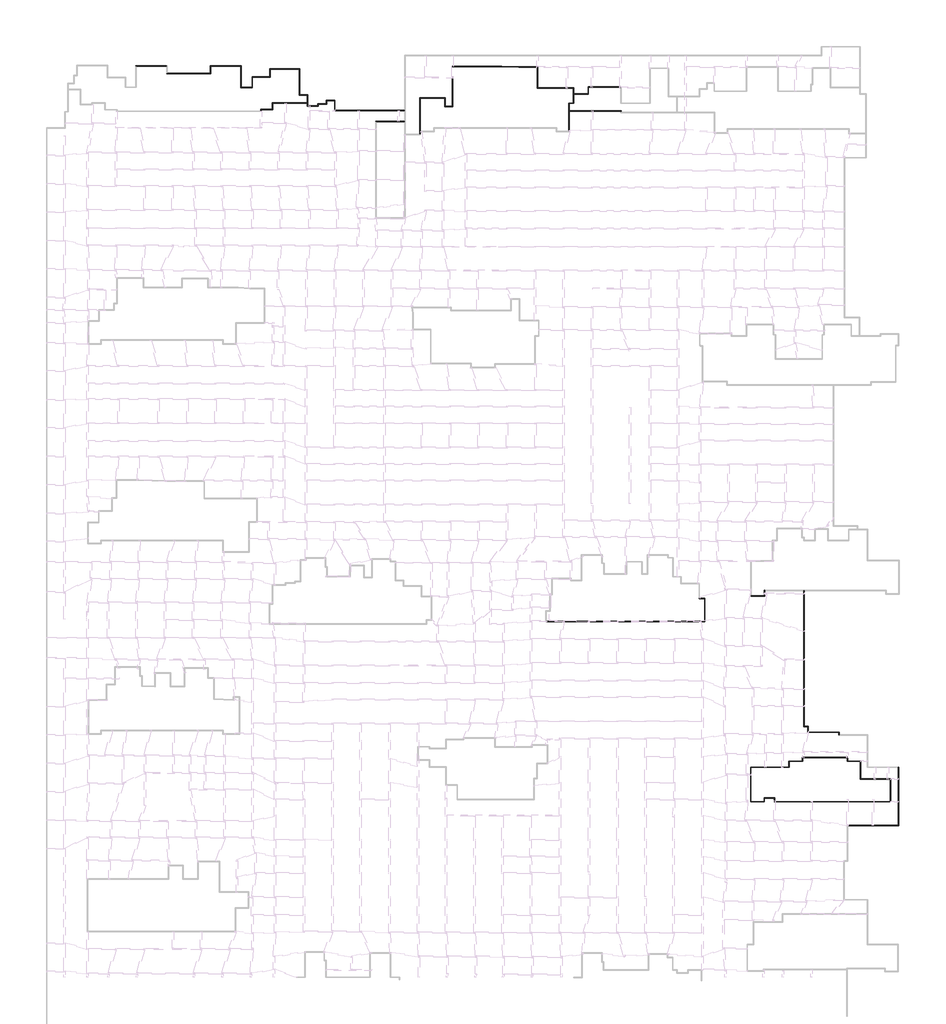
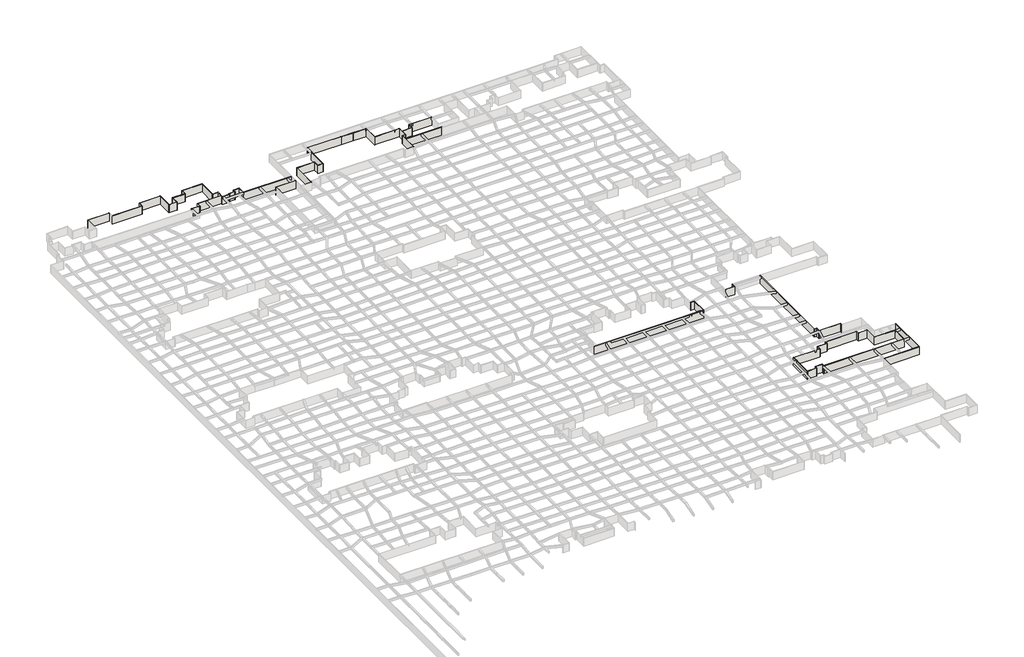
# One storey, part 8 of 45: 70 walls.
"""IFC4 building model written with IfcOpenShell, lengths in millimetres."""

from ifc_helpers import new_model, si_unit, origin, origin_with_axes, place, context, project, spatial, polyline, outline, extrude, faceted_brep, element, save

model = new_model("IFC4")

# Units and contexts
model_context = context("Model", 3, world=origin())
ifc_project = project(units=[si_unit("LENGTHUNIT", "METRE", prefix="MILLI")], contexts=[model_context])

# Site, building, storey
site = spatial("IfcSite", under=ifc_project)
building = spatial("IfcBuilding", under=site)
storey = spatial("IfcBuildingStorey", under=building, Name="户型图", Elevation=0.0)

# Walls
placement = place(None, origin())
element("IfcWall", 1, ObjectType="所有墙体", at=placement, inside=storey, context=model_context, shape_type="Brep", body=[
    faceted_brep([(64419.4783436, 211.9876735, 0.0), (78319.4783436, 211.9876735, 0.0), (78319.4783436, 211.9876735, 3300.0), (64419.4783436, 211.9876735, 3300.0), (64419.4783436, 331.9876735, 0.0), (64419.4783436, 331.9876735, 3300.0), (78199.4783436, 331.9876735, 3300.0), (78319.4783436, 331.9876735, 3300.0), (78319.4783436, 331.9876735, 0.0), (78199.4783436, 331.9876735, 0.0)], [[[0, 1, 2, 3]], [[4, 5, 6, 7, 8, 9]], [[1, 0, 4, 9, 8]], [[3, 2, 7, 6, 5]], [[0, 3, 5, 4]], [[2, 1, 8, 7]]]),
])
element("IfcWall", 2, ObjectType="所有墙体", at=placement, inside=storey, context=model_context, shape_type="Brep", body=[
    faceted_brep([(78319.4783436, 331.9876735, 0.0), (78319.4783436, 16231.9876735, 0.0), (78319.4783436, 16231.9876735, 3300.0), (78319.4783436, 331.9876735, 3300.0), (78199.4783436, 331.9876735, 0.0), (78199.4783436, 331.9876735, 3300.0), (78199.4783436, 16111.9876735, 3300.0), (78199.4783436, 16231.9876735, 3300.0), (78199.4783436, 16231.9876735, 0.0), (78199.4783436, 16111.9876735, 0.0)], [[[0, 1, 2, 3]], [[4, 5, 6, 7, 8, 9]], [[1, 0, 4, 9, 8]], [[3, 2, 7, 6, 5]], [[0, 3, 5, 4]], [[2, 1, 8, 7]]]),
])
element("IfcWall", 3, ObjectType="所有墙体", at=placement, inside=storey, context=model_context, shape_type="Brep", body=[
    faceted_brep([(62019.4783436, 25131.9876735, 0.0), (62019.4783436, 25831.9876735, 0.0), (62019.4783436, 25831.9876735, 3300.0), (62019.4783436, 25131.9876735, 3300.0), (61899.4783436, 25131.9876735, 0.0), (61899.4783436, 25131.9876735, 3300.0), (61899.4783436, 25711.9876735, 3300.0), (61899.4783436, 25831.9876735, 3300.0), (61899.4783436, 25831.9876735, 0.0), (61899.4783436, 25711.9876735, 0.0)], [[[0, 1, 2, 3]], [[4, 5, 6, 7, 8, 9]], [[1, 0, 4, 9, 8]], [[3, 2, 7, 6, 5]], [[0, 3, 5, 4]], [[2, 1, 8, 7]]]),
])
element("IfcWall", 4, ObjectType="所有墙体", at=placement, inside=storey, context=model_context, shape_type="Brep", body=[
    faceted_brep([(61899.4783436, 25831.9876735, 0.0), (53519.4783436, 25831.9876735, 0.0), (53399.4783436, 25831.9876735, 0.0), (53399.4783436, 25831.9876735, 3300.0), (53519.4783436, 25831.9876735, 3300.0), (61899.4783436, 25831.9876735, 3300.0), (61899.4783436, 25711.9876735, 0.0), (61899.4783436, 25711.9876735, 3300.0), (53399.4783436, 25711.9876735, 3300.0), (53399.4783436, 25711.9876735, 0.0)], [[[0, 1, 2, 3, 4, 5]], [[6, 7, 8, 9]], [[2, 1, 0, 6, 9]], [[5, 4, 3, 8, 7]], [[0, 5, 7, 6]], [[3, 2, 9, 8]]]),
])
element("IfcWall", 5, ObjectType="所有墙体", at=placement, inside=storey, context=model_context, shape_type="Brep", body=[
    faceted_brep([(53519.4783436, 25831.9876735, 0.0), (53519.4783436, 27431.9876735, 0.0), (53519.4783436, 27431.9876735, 3300.0), (53519.4783436, 25831.9876735, 3300.0), (53399.4783436, 25831.9876735, 0.0), (53399.4783436, 25831.9876735, 3300.0), (53399.4783436, 27311.9876735, 3300.0), (53399.4783436, 27431.9876735, 3300.0), (53399.4783436, 27431.9876735, 0.0), (53399.4783436, 27311.9876735, 0.0)], [[[0, 1, 2, 3]], [[4, 5, 6, 7, 8, 9]], [[1, 0, 4, 9, 8]], [[3, 2, 7, 6, 5]], [[0, 3, 5, 4]], [[2, 1, 8, 7]]]),
])
element("IfcWall", 6, ObjectType="所有墙体", at=placement, inside=storey, context=model_context, shape_type="Brep", body=[
    faceted_brep([(53399.4783436, 27431.9876735, 0.0), (52519.4783436, 27431.9876735, 0.0), (52399.4783436, 27431.9876735, 0.0), (52399.4783436, 27431.9876735, 3300.0), (52519.4783436, 27431.9876735, 3300.0), (53399.4783436, 27431.9876735, 3300.0), (53399.4783436, 27311.9876735, 0.0), (53399.4783436, 27311.9876735, 3300.0), (52399.4783436, 27311.9876735, 3300.0), (52399.4783436, 27311.9876735, 0.0)], [[[0, 1, 2, 3, 4, 5]], [[6, 7, 8, 9]], [[2, 1, 0, 6, 9]], [[5, 4, 3, 8, 7]], [[0, 5, 7, 6]], [[3, 2, 9, 8]]]),
])
element("IfcWall", 7, ObjectType="所有墙体", at=placement, inside=storey, context=model_context, shape_type="SweptSolid", body=[
    extrude(outline(polyline([(52519.4783436, 64511.9876735), (52519.4783436, 27431.9876735), (52399.4783436, 27431.9876735), (52399.4783436, 64511.9876735), (52519.4783436, 64511.9876735)])), origin_with_axes(), (0.0, 0.0, 1.0), 3300.0),
])
element("IfcWall", 8, ObjectType="所有墙体", at=placement, inside=storey, context=model_context, shape_type="Brep", body=[
    faceted_brep([(-57000.5216564, 196131.9876735, 0.0), (-76080.5216564, 196131.9876735, 0.0), (-76200.5216564, 196131.9876735, 0.0), (-76200.5216564, 196131.9876735, 3300.0), (-76080.5216564, 196131.9876735, 3300.0), (-57000.5216564, 196131.9876735, 3300.0), (-57000.5216564, 196011.9876735, 0.0), (-57000.5216564, 196011.9876735, 3300.0), (-76200.5216564, 196011.9876735, 3300.0), (-76200.5216564, 196011.9876735, 0.0)], [[[0, 1, 2, 3, 4, 5]], [[6, 7, 8, 9]], [[2, 1, 0, 6, 9]], [[5, 4, 3, 8, 7]], [[0, 5, 7, 6]], [[3, 2, 9, 8]]]),
])
element("IfcWall", 9, ObjectType="所有墙体", at=placement, inside=storey, context=model_context, shape_type="Brep", body=[
    faceted_brep([(-76080.5216564, 196131.9876735, 0.0), (-76080.5216564, 198931.9876735, 0.0), (-76080.5216564, 198931.9876735, 3300.0), (-76080.5216564, 196131.9876735, 3300.0), (-76200.5216564, 196131.9876735, 0.0), (-76200.5216564, 196131.9876735, 3300.0), (-76200.5216564, 198811.9876735, 3300.0), (-76200.5216564, 198931.9876735, 3300.0), (-76200.5216564, 198931.9876735, 0.0), (-76200.5216564, 198811.9876735, 0.0)], [[[0, 1, 2, 3]], [[4, 5, 6, 7, 8, 9]], [[1, 0, 4, 9, 8]], [[3, 2, 7, 6, 5]], [[0, 3, 5, 4]], [[2, 1, 8, 7]]]),
])
element("IfcWall", 10, ObjectType="所有墙体", at=placement, inside=storey, context=model_context, shape_type="Brep", body=[
    faceted_brep([(-76200.5216564, 198931.9876735, 0.0), (-78500.5216564, 198931.9876735, 0.0), (-78500.5216564, 198931.9876735, 3300.0), (-76200.5216564, 198931.9876735, 3300.0), (-76200.5216564, 198811.9876735, 0.0), (-76200.5216564, 198811.9876735, 3300.0), (-78380.5216564, 198811.9876735, 3300.0), (-78500.5216564, 198811.9876735, 3300.0), (-78500.5216564, 198811.9876735, 0.0), (-78380.5216564, 198811.9876735, 0.0)], [[[0, 1, 2, 3]], [[4, 5, 6, 7, 8, 9]], [[1, 0, 4, 9, 8]], [[3, 2, 7, 6, 5]], [[0, 3, 5, 4]], [[2, 1, 8, 7]]]),
])
element("IfcWall", 11, ObjectType="所有墙体", at=placement, inside=storey, context=model_context, shape_type="Brep", body=[
    faceted_brep([(-78500.5216564, 198811.9876735, 0.0), (-78500.5216564, 197931.9876735, 0.0), (-78500.5216564, 197811.9876735, 0.0), (-78500.5216564, 197811.9876735, 3300.0), (-78500.5216564, 197931.9876735, 3300.0), (-78500.5216564, 198811.9876735, 3300.0), (-78380.5216564, 198811.9876735, 0.0), (-78380.5216564, 198811.9876735, 3300.0), (-78380.5216564, 197811.9876735, 3300.0), (-78380.5216564, 197811.9876735, 0.0)], [[[0, 1, 2, 3, 4, 5]], [[6, 7, 8, 9]], [[2, 1, 0, 6, 9]], [[5, 4, 3, 8, 7]], [[0, 5, 7, 6]], [[3, 2, 9, 8]]]),
])
element("IfcWall", 12, ObjectType="所有墙体", at=placement, inside=storey, context=model_context, shape_type="Brep", body=[
    faceted_brep([(-78500.5216564, 197931.9876735, 0.0), (-80800.5216564, 197931.9876735, 0.0), (-80800.5216564, 197931.9876735, 3300.0), (-78500.5216564, 197931.9876735, 3300.0), (-78500.5216564, 197811.9876735, 0.0), (-78500.5216564, 197811.9876735, 3300.0), (-80680.5216564, 197811.9876735, 3300.0), (-80800.5216564, 197811.9876735, 3300.0), (-80800.5216564, 197811.9876735, 0.0), (-80680.5216564, 197811.9876735, 0.0)], [[[0, 1, 2, 3]], [[4, 5, 6, 7, 8, 9]], [[1, 0, 4, 9, 8]], [[3, 2, 7, 6, 5]], [[0, 3, 5, 4]], [[2, 1, 8, 7]]]),
])
element("IfcWall", 13, ObjectType="所有墙体", at=placement, inside=storey, context=model_context, shape_type="Brep", body=[
    faceted_brep([(-80800.5216564, 197811.9876735, 0.0), (-80800.5216564, 197431.9876735, 0.0), (-80800.5216564, 197311.9876735, 0.0), (-80800.5216564, 197311.9876735, 3300.0), (-80800.5216564, 197431.9876735, 3300.0), (-80800.5216564, 197811.9876735, 3300.0), (-80680.5216564, 197811.9876735, 0.0), (-80680.5216564, 197811.9876735, 3300.0), (-80680.5216564, 197311.9876735, 3300.0), (-80680.5216564, 197311.9876735, 0.0)], [[[0, 1, 2, 3, 4, 5]], [[6, 7, 8, 9]], [[2, 1, 0, 6, 9]], [[5, 4, 3, 8, 7]], [[0, 5, 7, 6]], [[3, 2, 9, 8]]]),
])
element("IfcWall", 14, ObjectType="所有墙体", at=placement, inside=storey, context=model_context, shape_type="Brep", body=[
    faceted_brep([(-80800.5216564, 197431.9876735, 0.0), (-83580.5216564, 197431.9876735, 0.0), (-83700.5216564, 197431.9876735, 0.0), (-83700.5216564, 197431.9876735, 3300.0), (-83580.5216564, 197431.9876735, 3300.0), (-80800.5216564, 197431.9876735, 3300.0), (-80800.5216564, 197311.9876735, 0.0), (-80800.5216564, 197311.9876735, 3300.0), (-83700.5216564, 197311.9876735, 3300.0), (-83700.5216564, 197311.9876735, 0.0)], [[[0, 1, 2, 3, 4, 5]], [[6, 7, 8, 9]], [[2, 1, 0, 6, 9]], [[5, 4, 3, 8, 7]], [[0, 5, 7, 6]], [[3, 2, 9, 8]]]),
])
element("IfcWall", 15, ObjectType="所有墙体", at=placement, inside=storey, context=model_context, shape_type="Brep", body=[
    faceted_brep([(-83580.5216564, 197431.9876735, 0.0), (-83580.5216564, 200431.9876735, 0.0), (-83580.5216564, 200431.9876735, 3300.0), (-83580.5216564, 197431.9876735, 3300.0), (-83700.5216564, 197431.9876735, 0.0), (-83700.5216564, 197431.9876735, 3300.0), (-83700.5216564, 198051.9876735, 3300.0), (-83700.5216564, 198171.9876735, 3300.0), (-83700.5216564, 200311.9876735, 3300.0), (-83700.5216564, 200431.9876735, 3300.0), (-83700.5216564, 200431.9876735, 0.0), (-83700.5216564, 200311.9876735, 0.0), (-83700.5216564, 198171.9876735, 0.0), (-83700.5216564, 198051.9876735, 0.0)], [[[0, 1, 2, 3]], [[4, 5, 6, 7, 8, 9, 10, 11, 12, 13]], [[1, 0, 4, 13, 12, 11, 10]], [[3, 2, 9, 8, 7, 6, 5]], [[2, 1, 10, 9]], [[0, 3, 5, 4]]]),
])
element("IfcWall", 16, ObjectType="所有墙体", at=placement, inside=storey, context=model_context, shape_type="Brep", body=[
    faceted_brep([(-83700.5216564, 200431.9876735, 0.0), (-85680.5216564, 200431.9876735, 0.0), (-85800.5216564, 200431.9876735, 0.0), (-85800.5216564, 200431.9876735, 3300.0), (-85680.5216564, 200431.9876735, 3300.0), (-83700.5216564, 200431.9876735, 3300.0), (-83700.5216564, 200311.9876735, 0.0), (-83700.5216564, 200311.9876735, 3300.0), (-85800.5216564, 200311.9876735, 3300.0), (-85800.5216564, 200311.9876735, 0.0)], [[[0, 1, 2, 3, 4, 5]], [[6, 7, 8, 9]], [[2, 1, 0, 6, 9]], [[5, 4, 3, 8, 7]], [[0, 5, 7, 6]], [[3, 2, 9, 8]]]),
])
element("IfcWall", 17, ObjectType="所有墙体", at=placement, inside=storey, context=model_context, shape_type="Brep", body=[
    faceted_brep([(-85680.5216564, 200431.9876735, 0.0), (-85680.5216564, 207531.9876735, 0.0), (-85680.5216564, 207531.9876735, 3300.0), (-85680.5216564, 200431.9876735, 3300.0), (-85800.5216564, 200431.9876735, 0.0), (-85800.5216564, 200431.9876735, 3300.0), (-85800.5216564, 207411.9876735, 3300.0), (-85800.5216564, 207531.9876735, 3300.0), (-85800.5216564, 207531.9876735, 0.0), (-85800.5216564, 207411.9876735, 0.0)], [[[0, 1, 2, 3]], [[4, 5, 6, 7, 8, 9]], [[1, 0, 4, 9, 8]], [[3, 2, 7, 6, 5]], [[0, 3, 5, 4]], [[2, 1, 8, 7]]]),
])
element("IfcWall", 18, ObjectType="所有墙体", at=placement, inside=storey, context=model_context, shape_type="Brep", body=[
    faceted_brep([(-85800.5216564, 207531.9876735, 0.0), (-93900.5216564, 207531.9876735, 0.0), (-93900.5216564, 207531.9876735, 3300.0), (-85800.5216564, 207531.9876735, 3300.0), (-85800.5216564, 207411.9876735, 0.0), (-85800.5216564, 207411.9876735, 3300.0), (-93780.5216564, 207411.9876735, 3300.0), (-93900.5216564, 207411.9876735, 3300.0), (-93900.5216564, 207411.9876735, 0.0), (-93780.5216564, 207411.9876735, 0.0)], [[[0, 1, 2, 3]], [[4, 5, 6, 7, 8, 9]], [[1, 0, 4, 9, 8]], [[3, 2, 7, 6, 5]], [[0, 3, 5, 4]], [[2, 1, 8, 7]]]),
])
element("IfcWall", 19, ObjectType="所有墙体", at=placement, inside=storey, context=model_context, shape_type="Brep", body=[
    faceted_brep([(-93900.5216564, 207411.9876735, 0.0), (-93900.5216564, 205331.9876735, 0.0), (-93900.5216564, 205211.9876735, 0.0), (-93900.5216564, 205211.9876735, 3300.0), (-93900.5216564, 205331.9876735, 3300.0), (-93900.5216564, 207411.9876735, 3300.0), (-93780.5216564, 207411.9876735, 0.0), (-93780.5216564, 207411.9876735, 3300.0), (-93780.5216564, 205211.9876735, 3300.0), (-93780.5216564, 205211.9876735, 0.0)], [[[0, 1, 2, 3, 4, 5]], [[6, 7, 8, 9]], [[2, 1, 0, 6, 9]], [[5, 4, 3, 8, 7]], [[0, 5, 7, 6]], [[3, 2, 9, 8]]]),
])
element("IfcWall", 20, ObjectType="所有墙体", at=placement, inside=storey, context=model_context, shape_type="Brep", body=[
    faceted_brep([(-93900.5216564, 205331.9876735, 0.0), (-98800.5216564, 205331.9876735, 0.0), (-98800.5216564, 205331.9876735, 3300.0), (-93900.5216564, 205331.9876735, 3300.0), (-93900.5216564, 205211.9876735, 0.0), (-93900.5216564, 205211.9876735, 3300.0), (-98680.5216564, 205211.9876735, 3300.0), (-98800.5216564, 205211.9876735, 3300.0), (-98800.5216564, 205211.9876735, 0.0), (-98680.5216564, 205211.9876735, 0.0)], [[[0, 1, 2, 3]], [[4, 5, 6, 7, 8, 9]], [[1, 0, 4, 9, 8]], [[3, 2, 7, 6, 5]], [[0, 3, 5, 4]], [[2, 1, 8, 7]]]),
])
element("IfcWall", 21, ObjectType="所有墙体", at=placement, inside=storey, context=model_context, shape_type="Brep", body=[
    faceted_brep([(-98800.5216564, 205211.9876735, 0.0), (-98800.5216564, 202431.9876735, 0.0), (-98800.5216564, 202311.9876735, 0.0), (-98800.5216564, 202311.9876735, 3300.0), (-98800.5216564, 202431.9876735, 3300.0), (-98800.5216564, 205211.9876735, 3300.0), (-98680.5216564, 205211.9876735, 0.0), (-98680.5216564, 205211.9876735, 3300.0), (-98680.5216564, 202311.9876735, 3300.0), (-98680.5216564, 202311.9876735, 0.0)], [[[0, 1, 2, 3, 4, 5]], [[6, 7, 8, 9]], [[2, 1, 0, 6, 9]], [[5, 4, 3, 8, 7]], [[0, 5, 7, 6]], [[3, 2, 9, 8]]]),
])
element("IfcWall", 22, ObjectType="所有墙体", at=placement, inside=storey, context=model_context, shape_type="Brep", body=[
    faceted_brep([(-98800.5216564, 202431.9876735, 0.0), (-101780.5216564, 202431.9876735, 0.0), (-101900.5216564, 202431.9876735, 0.0), (-101900.5216564, 202431.9876735, 3300.0), (-101780.5216564, 202431.9876735, 3300.0), (-98800.5216564, 202431.9876735, 3300.0), (-98800.5216564, 202311.9876735, 0.0), (-98800.5216564, 202311.9876735, 3300.0), (-101900.5216564, 202311.9876735, 3300.0), (-101900.5216564, 202311.9876735, 0.0)], [[[0, 1, 2, 3, 4, 5]], [[6, 7, 8, 9]], [[2, 1, 0, 6, 9]], [[5, 4, 3, 8, 7]], [[0, 5, 7, 6]], [[3, 2, 9, 8]]]),
])
element("IfcWall", 23, ObjectType="所有墙体", at=placement, inside=storey, context=model_context, shape_type="Brep", body=[
    faceted_brep([(-101780.5216564, 202431.9876735, 0.0), (-101780.5216564, 208331.9876735, 0.0), (-101780.5216564, 208331.9876735, 3300.0), (-101780.5216564, 202431.9876735, 3300.0), (-101900.5216564, 202431.9876735, 0.0), (-101900.5216564, 202431.9876735, 3300.0), (-101900.5216564, 208211.9876735, 3300.0), (-101900.5216564, 208331.9876735, 3300.0), (-101900.5216564, 208331.9876735, 0.0), (-101900.5216564, 208211.9876735, 0.0)], [[[0, 1, 2, 3]], [[4, 5, 6, 7, 8, 9]], [[1, 0, 4, 9, 8]], [[3, 2, 7, 6, 5]], [[0, 3, 5, 4]], [[2, 1, 8, 7]]]),
])
element("IfcWall", 24, ObjectType="所有墙体", at=placement, inside=storey, context=model_context, shape_type="Brep", body=[
    faceted_brep([(-101900.5216564, 208331.9876735, 0.0), (-110300.5216564, 208331.9876735, 0.0), (-110300.5216564, 208331.9876735, 3300.0), (-101900.5216564, 208331.9876735, 3300.0), (-101900.5216564, 208211.9876735, 0.0), (-101900.5216564, 208211.9876735, 3300.0), (-110180.5216564, 208211.9876735, 3300.0), (-110300.5216564, 208211.9876735, 3300.0), (-110300.5216564, 208211.9876735, 0.0), (-110180.5216564, 208211.9876735, 0.0)], [[[0, 1, 2, 3]], [[4, 5, 6, 7, 8, 9]], [[1, 0, 4, 9, 8]], [[3, 2, 7, 6, 5]], [[0, 3, 5, 4]], [[2, 1, 8, 7]]]),
])
element("IfcWall", 25, ObjectType="所有墙体", at=placement, inside=storey, context=model_context, shape_type="Brep", body=[
    faceted_brep([(-110300.5216564, 208211.9876735, 0.0), (-110300.5216564, 206331.9876735, 0.0), (-110300.5216564, 206211.9876735, 0.0), (-110300.5216564, 206211.9876735, 3300.0), (-110300.5216564, 206331.9876735, 3300.0), (-110300.5216564, 208211.9876735, 3300.0), (-110180.5216564, 208211.9876735, 0.0), (-110180.5216564, 208211.9876735, 3300.0), (-110180.5216564, 206211.9876735, 3300.0), (-110180.5216564, 206211.9876735, 0.0)], [[[0, 1, 2, 3, 4, 5]], [[6, 7, 8, 9]], [[2, 1, 0, 6, 9]], [[5, 4, 3, 8, 7]], [[0, 5, 7, 6]], [[3, 2, 9, 8]]]),
])
element("IfcWall", 26, ObjectType="所有墙体", at=placement, inside=storey, context=model_context, shape_type="Brep", body=[
    faceted_brep([(-110300.5216564, 206331.9876735, 0.0), (-121980.5216564, 206331.9876735, 0.0), (-122100.5216564, 206331.9876735, 0.0), (-122100.5216564, 206331.9876735, 3300.0), (-121980.5216564, 206331.9876735, 3300.0), (-110300.5216564, 206331.9876735, 3300.0), (-110300.5216564, 206211.9876735, 0.0), (-110300.5216564, 206211.9876735, 3300.0), (-122100.5216564, 206211.9876735, 3300.0), (-122100.5216564, 206211.9876735, 0.0)], [[[0, 1, 2, 3, 4, 5]], [[6, 7, 8, 9]], [[2, 1, 0, 6, 9]], [[5, 4, 3, 8, 7]], [[0, 5, 7, 6]], [[3, 2, 9, 8]]]),
])
element("IfcWall", 27, ObjectType="所有墙体", at=placement, inside=storey, context=model_context, shape_type="Brep", body=[
    faceted_brep([(-122100.5216564, 208331.9876735, 0.0), (-130600.5216564, 208331.9876735, 0.0), (-130600.5216564, 208331.9876735, 3300.0), (-122100.5216564, 208331.9876735, 3300.0), (-122100.5216564, 208211.9876735, 0.0), (-122100.5216564, 208211.9876735, 3300.0), (-130480.5216564, 208211.9876735, 3300.0), (-130600.5216564, 208211.9876735, 3300.0), (-130600.5216564, 208211.9876735, 0.0), (-130480.5216564, 208211.9876735, 0.0)], [[[0, 1, 2, 3]], [[4, 5, 6, 7, 8, 9]], [[1, 0, 4, 9, 8]], [[3, 2, 7, 6, 5]], [[0, 3, 5, 4]], [[2, 1, 8, 7]]]),
])
element("IfcWall", 28, ObjectType="所有墙体", at=placement, inside=storey, context=model_context, shape_type="Brep", body=[
    faceted_brep([(-96280.5216564, 195971.9876735, 0.0), (-96280.5216564, 196351.9876735, 0.0), (-96280.5216564, 196471.9876735, 0.0), (-96280.5216564, 196471.9876735, 3300.0), (-96280.5216564, 196351.9876735, 3300.0), (-96280.5216564, 195971.9876735, 3300.0), (-96400.5216564, 195971.9876735, 0.0), (-96400.5216564, 195971.9876735, 3300.0), (-96400.5216564, 196471.9876735, 3300.0), (-96400.5216564, 196471.9876735, 0.0)], [[[0, 1, 2, 3, 4, 5]], [[6, 7, 8, 9]], [[2, 1, 0, 6, 9]], [[5, 4, 3, 8, 7]], [[0, 5, 7, 6]], [[3, 2, 9, 8]]]),
])
element("IfcWall", 29, ObjectType="所有墙体", at=placement, inside=storey, context=model_context, shape_type="Brep", body=[
    faceted_brep([(-96280.5216564, 196351.9876735, 0.0), (-93080.5216564, 196351.9876735, 0.0), (-93080.5216564, 196351.9876735, 3300.0), (-96280.5216564, 196351.9876735, 3300.0), (-96280.5216564, 196471.9876735, 0.0), (-96280.5216564, 196471.9876735, 3300.0), (-93200.5216564, 196471.9876735, 3300.0), (-93080.5216564, 196471.9876735, 3300.0), (-93080.5216564, 196471.9876735, 0.0), (-93200.5216564, 196471.9876735, 0.0)], [[[0, 1, 2, 3]], [[4, 5, 6, 7, 8, 9]], [[1, 0, 4, 9, 8]], [[3, 2, 7, 6, 5]], [[0, 3, 5, 4]], [[2, 1, 8, 7]]]),
])
element("IfcWall", 30, ObjectType="所有墙体", at=placement, inside=storey, context=model_context, shape_type="Brep", body=[
    faceted_brep([(-93080.5216564, 196471.9876735, 0.0), (-93080.5216564, 198051.9876735, 0.0), (-93080.5216564, 198171.9876735, 0.0), (-93080.5216564, 198171.9876735, 3300.0), (-93080.5216564, 198051.9876735, 3300.0), (-93080.5216564, 196471.9876735, 3300.0), (-93200.5216564, 196471.9876735, 0.0), (-93200.5216564, 196471.9876735, 3300.0), (-93200.5216564, 198171.9876735, 3300.0), (-93200.5216564, 198171.9876735, 0.0)], [[[0, 1, 2, 3, 4, 5]], [[6, 7, 8, 9]], [[2, 1, 0, 6, 9]], [[5, 4, 3, 8, 7]], [[0, 5, 7, 6]], [[3, 2, 9, 8]]]),
])
element("IfcWall", 31, ObjectType="所有墙体", at=placement, inside=storey, context=model_context, shape_type="SweptSolid", body=[
    extrude(outline(polyline([(-83700.5216564, 198051.9876735), (-93080.5216564, 198051.9876735), (-93080.5216564, 198171.9876735), (-83700.5216564, 198171.9876735), (-83700.5216564, 198051.9876735)])), origin_with_axes(), (0.0, 0.0, 1.0), 3300.0),
])
element("IfcWall", 32, ObjectType="所有墙体", at=placement, inside=storey, context=model_context, shape_type="Brep", body=[
    faceted_brep([(-64862.224124, 193082.3986126, 0.0), (-64742.224124, 193082.3986126, 0.0), (-57000.5216564, 193082.3986126, 0.0), (-57000.5216564, 193082.3986126, 3300.0), (-64742.224124, 193082.3986126, 3300.0), (-64862.224124, 193082.3986126, 3300.0), (-64862.224124, 193202.3986126, 0.0), (-64862.224124, 193202.3986126, 3300.0), (-57000.5216564, 193202.3986126, 3300.0), (-57000.5216564, 193202.3986126, 0.0)], [[[0, 1, 2, 3, 4, 5]], [[6, 7, 8, 9]], [[2, 1, 0, 6, 9]], [[5, 4, 3, 8, 7]], [[3, 2, 9, 8]], [[0, 5, 7, 6]]]),
])
element("IfcWall", 33, ObjectType="所有墙体", at=placement, inside=storey, context=model_context, shape_type="Brep", body=[
    faceted_brep([(-52780.5216564, 189542.3986126, 0.0), (-52780.5216564, 190322.3986126, 0.0), (-52780.5216564, 190442.3986126, 0.0), (-52780.5216564, 199430.8795616, 0.0), (-52780.5216564, 199430.8795616, 3300.0), (-52780.5216564, 190442.3986126, 3300.0), (-52780.5216564, 190322.3986126, 3300.0), (-52780.5216564, 189542.3986126, 3300.0), (-52900.5216564, 189542.3986126, 0.0), (-52900.5216564, 189542.3986126, 3300.0), (-52900.5216564, 199430.8795616, 3300.0), (-52900.5216564, 199430.8795616, 0.0)], [[[0, 1, 2, 3, 4, 5, 6, 7]], [[8, 9, 10, 11]], [[3, 2, 1, 0, 8, 11]], [[7, 6, 5, 4, 10, 9]], [[0, 7, 9, 8]], [[4, 3, 11, 10]]]),
])
element("IfcWall", 34, ObjectType="所有墙体", at=placement, inside=storey, context=model_context, shape_type="Brep", body=[
    faceted_brep([(-11926.7821096, 190442.3986126, 0.0), (-11926.7821096, 195871.9680247, 0.0), (-11926.7821096, 195991.9680247, 0.0), (-11926.7821096, 198031.9680247, 0.0), (-11926.7821096, 198031.9680247, 3300.0), (-11926.7821096, 195991.9680247, 3300.0), (-11926.7821096, 195871.9680247, 3300.0), (-11926.7821096, 190442.3986126, 3300.0), (-12046.7821096, 190442.3986126, 0.0), (-12046.7821096, 190442.3986126, 3300.0), (-12046.7821096, 198031.9680247, 3300.0), (-12046.7821096, 198031.9680247, 0.0)], [[[0, 1, 2, 3, 4, 5, 6, 7]], [[8, 9, 10, 11]], [[3, 2, 1, 0, 8, 11]], [[7, 6, 5, 4, 10, 9]], [[0, 7, 9, 8]], [[4, 3, 11, 10]]]),
])
element("IfcWall", 35, ObjectType="所有墙体", at=placement, inside=storey, context=model_context, shape_type="Brep", body=[
    faceted_brep([(-11926.7821096, 195871.9680247, 0.0), (2251.0399311, 195871.9680247, 0.0), (2371.0399311, 195871.9680247, 0.0), (2371.0399311, 195871.9680247, 3300.0), (2251.0399311, 195871.9680247, 3300.0), (-11926.7821096, 195871.9680247, 3300.0), (-11926.7821096, 195991.9680247, 0.0), (-11926.7821096, 195991.9680247, 3300.0), (2371.0399311, 195991.9680247, 3300.0), (2371.0399311, 195991.9680247, 0.0)], [[[0, 1, 2, 3, 4, 5]], [[6, 7, 8, 9]], [[2, 1, 0, 6, 9]], [[5, 4, 3, 8, 7]], [[0, 5, 7, 6]], [[3, 2, 9, 8]]]),
])
element("IfcWall", 36, ObjectType="所有墙体", at=placement, inside=storey, context=model_context, shape_type="SweptSolid", body=[
    extrude(outline(polyline([(-30381.5689603, 208121.4336176), (-43880.5216564, 208121.4336176), (-43880.5216564, 208241.4336176), (-30379.4743525, 208241.4336176), (-30381.5689603, 208121.4336176)])), origin_with_axes(), (0.0, 0.0, 1.0), 3300.0),
])
element("IfcWall", 37, ObjectType="所有墙体", at=placement, inside=storey, context=model_context, shape_type="SweptSolid", body=[
    extrude(outline(polyline([(-25784.3711561, 207960.8959327), (-30381.5689603, 208121.4336176), (-30379.4743525, 208241.4336176), (-25782.2765483, 208080.8959327), (-25784.3711561, 207960.8959327)])), origin_with_axes(), (0.0, 0.0, 1.0), 3300.0),
])
element("IfcWall", 38, ObjectType="所有墙体", at=placement, inside=storey, context=model_context, shape_type="Brep", body=[
    faceted_brep([(-25784.3711561, 207960.8959327, 0.0), (-20643.3238522, 207960.8959327, 0.0), (-20523.3238522, 207960.8959327, 0.0), (-20523.3238522, 207960.8959327, 3300.0), (-20643.3238522, 207960.8959327, 3300.0), (-25784.3711561, 207960.8959327, 3300.0), (-25782.2765483, 208080.8959327, 0.0), (-25782.2765483, 208080.8959327, 3300.0), (-20523.3238522, 208080.8959327, 3300.0), (-20523.3238522, 208080.8959327, 0.0)], [[[0, 1, 2, 3, 4, 5]], [[6, 7, 8, 9]], [[2, 1, 0, 6, 9]], [[5, 4, 3, 8, 7]], [[0, 5, 7, 6]], [[3, 2, 9, 8]]]),
])
element("IfcWall", 39, ObjectType="所有墙体", at=placement, inside=storey, context=model_context, shape_type="Brep", body=[
    faceted_brep([(-20643.3238522, 207960.8959327, 0.0), (-20643.3238522, 202160.8959327, 0.0), (-20643.3238522, 202160.8959327, 3300.0), (-20643.3238522, 207960.8959327, 3300.0), (-20523.3238522, 207960.8959327, 0.0), (-20523.3238522, 207960.8959327, 3300.0), (-20523.3238522, 202280.8959327, 3300.0), (-20523.3238522, 202160.8959327, 3300.0), (-20523.3238522, 202160.8959327, 0.0), (-20523.3238522, 202280.8959327, 0.0)], [[[0, 1, 2, 3]], [[4, 5, 6, 7, 8, 9]], [[1, 0, 4, 9, 8]], [[3, 2, 7, 6, 5]], [[0, 3, 5, 4]], [[2, 1, 8, 7]]]),
])
element("IfcWall", 40, ObjectType="所有墙体", at=placement, inside=storey, context=model_context, shape_type="Brep", body=[
    faceted_brep([(-20523.3238522, 202160.8959327, 0.0), (-10843.3238522, 202160.8959327, 0.0), (-10723.3238522, 202160.8959327, 0.0), (-10723.3238522, 202160.8959327, 3300.0), (-10843.3238522, 202160.8959327, 3300.0), (-20523.3238522, 202160.8959327, 3300.0), (-20523.3238522, 202280.8959327, 0.0), (-20523.3238522, 202280.8959327, 3300.0), (-10723.3238522, 202280.8959327, 3300.0), (-10723.3238522, 202280.8959327, 0.0)], [[[0, 1, 2, 3, 4, 5]], [[6, 7, 8, 9]], [[2, 1, 0, 6, 9]], [[5, 4, 3, 8, 7]], [[0, 5, 7, 6]], [[3, 2, 9, 8]]]),
])
element("IfcWall", 41, ObjectType="所有墙体", at=placement, inside=storey, context=model_context, shape_type="Brep", body=[
    faceted_brep([(-10843.3238522, 202160.8959327, 0.0), (-10843.3238522, 198151.9680247, 0.0), (-10843.3238522, 198031.9680247, 0.0), (-10843.3238522, 198031.9680247, 3300.0), (-10843.3238522, 198151.9680247, 3300.0), (-10843.3238522, 202160.8959327, 3300.0), (-10723.3238522, 202160.8959327, 0.0), (-10723.3238522, 202160.8959327, 3300.0), (-10723.3238522, 200651.9680247, 3300.0), (-10723.3238522, 200531.9680247, 3300.0), (-10723.3238522, 198031.9680247, 3300.0), (-10723.3238522, 198031.9680247, 0.0), (-10723.3238522, 200531.9680247, 0.0), (-10723.3238522, 200651.9680247, 0.0)], [[[0, 1, 2, 3, 4, 5]], [[6, 7, 8, 9, 10, 11, 12, 13]], [[2, 1, 0, 6, 13, 12, 11]], [[5, 4, 3, 10, 9, 8, 7]], [[0, 5, 7, 6]], [[3, 2, 11, 10]]]),
])
element("IfcWall", 42, ObjectType="所有墙体", at=placement, inside=storey, context=model_context, shape_type="Brep", body=[
    faceted_brep([(-10843.3238522, 198151.9680247, 0.0), (-12046.7821096, 198151.9680247, 0.0), (-12046.7821096, 198151.9680247, 3300.0), (-10843.3238522, 198151.9680247, 3300.0), (-10843.3238522, 198031.9680247, 0.0), (-10843.3238522, 198031.9680247, 3300.0), (-11926.7821096, 198031.9680247, 3300.0), (-12046.7821096, 198031.9680247, 3300.0), (-12046.7821096, 198031.9680247, 0.0), (-11926.7821096, 198031.9680247, 0.0)], [[[0, 1, 2, 3]], [[4, 5, 6, 7, 8, 9]], [[1, 0, 4, 9, 8]], [[3, 2, 7, 6, 5]], [[0, 3, 5, 4]], [[2, 1, 8, 7]]]),
])
element("IfcWall", 43, ObjectType="所有墙体", at=placement, inside=storey, context=model_context, shape_type="Brep", body=[
    faceted_brep([(-43940.8233714, 205190.8795616, 0.0), (-43940.8233714, 197250.8795616, 0.0), (-43940.8233714, 197130.8795616, 0.0), (-43940.8233714, 197130.8795616, 3300.0), (-43940.8233714, 197250.8795616, 3300.0), (-43940.8233714, 205190.8795616, 3300.0), (-43820.8233714, 205190.8795616, 0.0), (-43820.8233714, 205190.8795616, 3300.0), (-43820.8233714, 197130.8795616, 3300.0), (-43820.8233714, 197130.8795616, 0.0)], [[[0, 1, 2, 3, 4, 5]], [[6, 7, 8, 9]], [[2, 1, 0, 6, 9]], [[5, 4, 3, 8, 7]], [[0, 5, 7, 6]], [[3, 2, 9, 8]]]),
])
element("IfcWall", 44, ObjectType="所有墙体", at=placement, inside=storey, context=model_context, shape_type="Brep", body=[
    faceted_brep([(-43940.8233714, 197250.8795616, 0.0), (-45920.8233714, 197250.8795616, 0.0), (-46040.8233714, 197250.8795616, 0.0), (-46040.8233714, 197250.8795616, 3300.0), (-45920.8233714, 197250.8795616, 3300.0), (-43940.8233714, 197250.8795616, 3300.0), (-43940.8233714, 197130.8795616, 0.0), (-43940.8233714, 197130.8795616, 3300.0), (-46040.8233714, 197130.8795616, 3300.0), (-46040.8233714, 197130.8795616, 0.0)], [[[0, 1, 2, 3, 4, 5]], [[6, 7, 8, 9]], [[2, 1, 0, 6, 9]], [[5, 4, 3, 8, 7]], [[0, 5, 7, 6]], [[3, 2, 9, 8]]]),
])
element("IfcWall", 45, ObjectType="所有墙体", at=placement, inside=storey, context=model_context, shape_type="Brep", body=[
    faceted_brep([(-45920.8233714, 197250.8795616, 0.0), (-45920.8233714, 199550.8795616, 0.0), (-45920.8233714, 199550.8795616, 3300.0), (-45920.8233714, 197250.8795616, 3300.0), (-46040.8233714, 197250.8795616, 0.0), (-46040.8233714, 197250.8795616, 3300.0), (-46040.8233714, 199430.8795616, 3300.0), (-46040.8233714, 199550.8795616, 3300.0), (-46040.8233714, 199550.8795616, 0.0), (-46040.8233714, 199430.8795616, 0.0)], [[[0, 1, 2, 3]], [[4, 5, 6, 7, 8, 9]], [[1, 0, 4, 9, 8]], [[3, 2, 7, 6, 5]], [[0, 3, 5, 4]], [[2, 1, 8, 7]]]),
])
element("IfcWall", 46, ObjectType="所有墙体", at=placement, inside=storey, context=model_context, shape_type="Brep", body=[
    faceted_brep([(-46040.8233714, 199550.8795616, 0.0), (-52900.5216564, 199550.8795616, 0.0), (-52900.5216564, 199550.8795616, 3300.0), (-46040.8233714, 199550.8795616, 3300.0), (-46040.8233714, 199430.8795616, 0.0), (-46040.8233714, 199430.8795616, 3300.0), (-52780.5216564, 199430.8795616, 3300.0), (-52900.5216564, 199430.8795616, 3300.0), (-52900.5216564, 199430.8795616, 0.0), (-52780.5216564, 199430.8795616, 0.0)], [[[0, 1, 2, 3]], [[4, 5, 6, 7, 8, 9]], [[1, 0, 4, 9, 8]], [[3, 2, 7, 6, 5]], [[0, 3, 5, 4]], [[2, 1, 8, 7]]]),
])
element("IfcWall", 47, ObjectType="所有墙体", at=placement, inside=storey, context=model_context, shape_type="Brep", body=[
    faceted_brep([(2251.0399311, 202651.9680247, 0.0), (-6748.9600689, 202651.9680247, 0.0), (-6748.9600689, 202651.9680247, 3300.0), (2251.0399311, 202651.9680247, 3300.0), (2251.0399311, 202531.9680247, 0.0), (2251.0399311, 202531.9680247, 3300.0), (-6628.9600689, 202531.9680247, 3300.0), (-6748.9600689, 202531.9680247, 3300.0), (-6748.9600689, 202531.9680247, 0.0), (-6628.9600689, 202531.9680247, 0.0)], [[[0, 1, 2, 3]], [[4, 5, 6, 7, 8, 9]], [[1, 0, 4, 9, 8]], [[3, 2, 7, 6, 5]], [[0, 3, 5, 4]], [[2, 1, 8, 7]]]),
])
element("IfcWall", 48, ObjectType="所有墙体", at=placement, inside=storey, context=model_context, shape_type="Brep", body=[
    faceted_brep([(-6748.9600689, 202531.9680247, 0.0), (-6748.9600689, 200651.9680247, 0.0), (-6748.9600689, 200531.9680247, 0.0), (-6748.9600689, 200531.9680247, 3300.0), (-6748.9600689, 200651.9680247, 3300.0), (-6748.9600689, 202531.9680247, 3300.0), (-6628.9600689, 202531.9680247, 0.0), (-6628.9600689, 202531.9680247, 3300.0), (-6628.9600689, 200531.9680247, 3300.0), (-6628.9600689, 200531.9680247, 0.0)], [[[0, 1, 2, 3, 4, 5]], [[6, 7, 8, 9]], [[2, 1, 0, 6, 9]], [[5, 4, 3, 8, 7]], [[0, 5, 7, 6]], [[3, 2, 9, 8]]]),
])
element("IfcWall", 49, ObjectType="所有墙体", at=placement, inside=storey, context=model_context, shape_type="SweptSolid", body=[
    extrude(outline(polyline([(-10723.3238522, 200651.9680247), (-6748.9600689, 200651.9680247), (-6748.9600689, 200531.9680247), (-10723.3238522, 200531.9680247), (-10723.3238522, 200651.9680247)])), origin_with_axes(), (0.0, 0.0, 1.0), 3300.0),
])
element("IfcWall", 50, ObjectType="所有墙体", at=placement, inside=storey, context=model_context, shape_type="Brep", body=[
    faceted_brep([(37907.3862954, 63018.4446559, 0.0), (41607.3862954, 63018.4446559, 0.0), (41607.3862954, 63018.4446559, 3300.0), (37907.3862954, 63018.4446559, 3300.0), (37907.3862954, 63138.4446559, 0.0), (37907.3862954, 63138.4446559, 3300.0), (41487.3862954, 63138.4446559, 3300.0), (41607.3862954, 63138.4446559, 3300.0), (41607.3862954, 63138.4446559, 0.0), (41487.3862954, 63138.4446559, 0.0)], [[[0, 1, 2, 3]], [[4, 5, 6, 7, 8, 9]], [[1, 0, 4, 9, 8]], [[3, 2, 7, 6, 5]], [[0, 3, 5, 4]], [[2, 1, 8, 7]]]),
])
element("IfcWall", 51, ObjectType="所有墙体", at=placement, inside=storey, context=model_context, shape_type="Brep", body=[
    faceted_brep([(41607.3862954, 63138.4446559, 0.0), (41607.3862954, 64511.9876735, 0.0), (41607.3862954, 64631.9876735, 0.0), (41607.3862954, 64631.9876735, 3300.0), (41607.3862954, 64511.9876735, 3300.0), (41607.3862954, 63138.4446559, 3300.0), (41487.3862954, 63138.4446559, 0.0), (41487.3862954, 63138.4446559, 3300.0), (41487.3862954, 64631.9876735, 3300.0), (41487.3862954, 64631.9876735, 0.0)], [[[0, 1, 2, 3, 4, 5]], [[6, 7, 8, 9]], [[2, 1, 0, 6, 9]], [[5, 4, 3, 8, 7]], [[0, 5, 7, 6]], [[3, 2, 9, 8]]]),
])
element("IfcWall", 52, ObjectType="所有墙体", at=placement, inside=storey, context=model_context, shape_type="Brep", body=[
    faceted_brep([(-18212.8482451, 56016.5180379, 0.0), (25287.1517549, 56016.5180379, 0.0), (25287.1517549, 56016.5180379, 3300.0), (-18212.8482451, 56016.5180379, 3300.0), (-18212.8482451, 56136.5180379, 0.0), (-18212.8482451, 56136.5180379, 3300.0), (25167.1517549, 56136.5180379, 3300.0), (25287.1517549, 56136.5180379, 3300.0), (25287.1517549, 56136.5180379, 0.0), (25167.1517549, 56136.5180379, 0.0)], [[[0, 1, 2, 3]], [[4, 5, 6, 7, 8, 9]], [[1, 0, 4, 9, 8]], [[3, 2, 7, 6, 5]], [[0, 3, 5, 4]], [[2, 1, 8, 7]]]),
])
element("IfcWall", 53, ObjectType="所有墙体", at=placement, inside=storey, context=model_context, shape_type="Brep", body=[
    faceted_brep([(25287.1517549, 56136.5180379, 0.0), (25287.1517549, 62436.5180379, 0.0), (25287.1517549, 62436.5180379, 3300.0), (25287.1517549, 56136.5180379, 3300.0), (25167.1517549, 56136.5180379, 0.0), (25167.1517549, 56136.5180379, 3300.0), (25167.1517549, 62316.5180379, 3300.0), (25167.1517549, 62436.5180379, 3300.0), (25167.1517549, 62436.5180379, 0.0), (25167.1517549, 62316.5180379, 0.0)], [[[0, 1, 2, 3]], [[4, 5, 6, 7, 8, 9]], [[1, 0, 4, 9, 8]], [[3, 2, 7, 6, 5]], [[0, 3, 5, 4]], [[2, 1, 8, 7]]]),
])
element("IfcWall", 54, ObjectType="所有墙体", at=placement, inside=storey, context=model_context, shape_type="Brep", body=[
    faceted_brep([(25167.1517549, 62436.5180379, 0.0), (23787.5629112, 62436.5180379, 0.0), (23667.5629112, 62436.5180379, 0.0), (23667.5629112, 62436.5180379, 3300.0), (23787.5629112, 62436.5180379, 3300.0), (25167.1517549, 62436.5180379, 3300.0), (25167.1517549, 62316.5180379, 0.0), (25167.1517549, 62316.5180379, 3300.0), (23667.5629112, 62316.5180379, 3300.0), (23667.5629112, 62316.5180379, 0.0)], [[[0, 1, 2, 3, 4, 5]], [[6, 7, 8, 9]], [[2, 1, 0, 6, 9]], [[5, 4, 3, 8, 7]], [[0, 5, 7, 6]], [[3, 2, 9, 8]]]),
])
element("IfcWall", 55, ObjectType="所有墙体", at=placement, inside=storey, context=model_context, shape_type="Brep", body=[
    faceted_brep([(37769.0116864, 16231.9876735, 0.0), (37769.0116864, 6667.4151595, 0.0), (37769.0116864, 6667.4151595, 3300.0), (37769.0116864, 16231.9876735, 3300.0), (37889.0116864, 16231.9876735, 0.0), (37889.0116864, 16231.9876735, 3300.0), (37889.0116864, 16111.9876735, 3300.0), (37889.0116864, 6787.4151595, 3300.0), (37889.0116864, 6667.4151595, 3300.0), (37889.0116864, 6667.4151595, 0.0), (37889.0116864, 6787.4151595, 0.0), (37889.0116864, 16111.9876735, 0.0)], [[[0, 1, 2, 3]], [[4, 5, 6, 7, 8, 9, 10, 11]], [[1, 0, 4, 11, 10, 9]], [[3, 2, 8, 7, 6, 5]], [[2, 1, 9, 8]], [[0, 3, 5, 4]]]),
])
element("IfcWall", 56, ObjectType="所有墙体", at=placement, inside=storey, context=model_context, shape_type="Brep", body=[
    faceted_brep([(37889.0116864, 6667.4151595, 0.0), (41589.0116864, 6667.4151595, 0.0), (41589.0116864, 6667.4151595, 3300.0), (37889.0116864, 6667.4151595, 3300.0), (37889.0116864, 6787.4151595, 0.0), (37889.0116864, 6787.4151595, 3300.0), (41469.0116864, 6787.4151595, 3300.0), (41589.0116864, 6787.4151595, 3300.0), (41589.0116864, 6787.4151595, 0.0), (41469.0116864, 6787.4151595, 0.0)], [[[0, 1, 2, 3]], [[4, 5, 6, 7, 8, 9]], [[1, 0, 4, 9, 8]], [[3, 2, 7, 6, 5]], [[0, 3, 5, 4]], [[2, 1, 8, 7]]]),
])
element("IfcWall", 57, ObjectType="所有墙体", at=placement, inside=storey, context=model_context, shape_type="Brep", body=[
    faceted_brep([(41589.0116864, 6787.4151595, 0.0), (41589.0116864, 7667.4151595, 0.0), (41589.0116864, 7787.4151595, 0.0), (41589.0116864, 7787.4151595, 3300.0), (41589.0116864, 7667.4151595, 3300.0), (41589.0116864, 6787.4151595, 3300.0), (41469.0116864, 6787.4151595, 0.0), (41469.0116864, 6787.4151595, 3300.0), (41469.0116864, 7787.4151595, 3300.0), (41469.0116864, 7787.4151595, 0.0)], [[[0, 1, 2, 3, 4, 5]], [[6, 7, 8, 9]], [[2, 1, 0, 6, 9]], [[5, 4, 3, 8, 7]], [[0, 5, 7, 6]], [[3, 2, 9, 8]]]),
])
element("IfcWall", 58, ObjectType="所有墙体", at=placement, inside=storey, context=model_context, shape_type="Brep", body=[
    faceted_brep([(41589.0116864, 7667.4151595, 0.0), (44269.0116864, 7667.4151595, 0.0), (44389.0116864, 7667.4151595, 0.0), (44389.0116864, 7667.4151595, 3300.0), (44269.0116864, 7667.4151595, 3300.0), (41589.0116864, 7667.4151595, 3300.0), (41589.0116864, 7787.4151595, 0.0), (41589.0116864, 7787.4151595, 3300.0), (44389.0116864, 7787.4151595, 3300.0), (44389.0116864, 7787.4151595, 0.0)], [[[0, 1, 2, 3, 4, 5]], [[6, 7, 8, 9]], [[2, 1, 0, 6, 9]], [[5, 4, 3, 8, 7]], [[0, 5, 7, 6]], [[3, 2, 9, 8]]]),
])
element("IfcWall", 59, ObjectType="所有墙体", at=placement, inside=storey, context=model_context, shape_type="Brep", body=[
    faceted_brep([(44269.0116864, 7667.4151595, 0.0), (44269.0116864, 6667.4151595, 0.0), (44269.0116864, 6667.4151595, 3300.0), (44269.0116864, 7667.4151595, 3300.0), (44389.0116864, 7667.4151595, 0.0), (44389.0116864, 7667.4151595, 3300.0), (44389.0116864, 6787.4151595, 3300.0), (44389.0116864, 6667.4151595, 3300.0), (44389.0116864, 6667.4151595, 0.0), (44389.0116864, 6787.4151595, 0.0)], [[[0, 1, 2, 3]], [[4, 5, 6, 7, 8, 9]], [[1, 0, 4, 9, 8]], [[3, 2, 7, 6, 5]], [[0, 3, 5, 4]], [[2, 1, 8, 7]]]),
])
element("IfcWall", 60, ObjectType="所有墙体", at=placement, inside=storey, context=model_context, shape_type="Brep", body=[
    faceted_brep([(44389.0116864, 6667.4151595, 0.0), (76189.0116864, 6667.4151595, 0.0), (76189.0116864, 6667.4151595, 3300.0), (44389.0116864, 6667.4151595, 3300.0), (44389.0116864, 6787.4151595, 0.0), (44389.0116864, 6787.4151595, 3300.0), (76069.0116864, 6787.4151595, 3300.0), (76189.0116864, 6787.4151595, 3300.0), (76189.0116864, 6787.4151595, 0.0), (76069.0116864, 6787.4151595, 0.0)], [[[0, 1, 2, 3]], [[4, 5, 6, 7, 8, 9]], [[1, 0, 4, 9, 8]], [[3, 2, 7, 6, 5]], [[0, 3, 5, 4]], [[2, 1, 8, 7]]]),
])
element("IfcWall", 61, ObjectType="所有墙体", at=placement, inside=storey, context=model_context, shape_type="Brep", body=[
    faceted_brep([(76189.0116864, 6787.4151595, 0.0), (76189.0116864, 12987.4151595, 0.0), (76189.0116864, 12987.4151595, 3300.0), (76189.0116864, 6787.4151595, 3300.0), (76069.0116864, 6787.4151595, 0.0), (76069.0116864, 6787.4151595, 3300.0), (76069.0116864, 12867.4151595, 3300.0), (76069.0116864, 12987.4151595, 3300.0), (76069.0116864, 12987.4151595, 0.0), (76069.0116864, 12867.4151595, 0.0)], [[[0, 1, 2, 3]], [[4, 5, 6, 7, 8, 9]], [[1, 0, 4, 9, 8]], [[3, 2, 7, 6, 5]], [[0, 3, 5, 4]], [[2, 1, 8, 7]]]),
])
element("IfcWall", 62, ObjectType="所有墙体", at=placement, inside=storey, context=model_context, shape_type="Brep", body=[
    faceted_brep([(76069.0116864, 12987.4151595, 0.0), (67989.0116864, 12987.4151595, 0.0), (67869.0116864, 12987.4151595, 0.0), (67869.0116864, 12987.4151595, 3300.0), (67989.0116864, 12987.4151595, 3300.0), (76069.0116864, 12987.4151595, 3300.0), (76069.0116864, 12867.4151595, 0.0), (76069.0116864, 12867.4151595, 3300.0), (67869.0116864, 12867.4151595, 3300.0), (67869.0116864, 12867.4151595, 0.0)], [[[0, 1, 2, 3, 4, 5]], [[6, 7, 8, 9]], [[2, 1, 0, 6, 9]], [[5, 4, 3, 8, 7]], [[0, 5, 7, 6]], [[3, 2, 9, 8]]]),
])
element("IfcWall", 63, ObjectType="所有墙体", at=placement, inside=storey, context=model_context, shape_type="Brep", body=[
    faceted_brep([(67989.0116864, 12987.4151595, 0.0), (67989.0116864, 17887.4151595, 0.0), (67989.0116864, 17887.4151595, 3300.0), (67989.0116864, 12987.4151595, 3300.0), (67869.0116864, 12987.4151595, 0.0), (67869.0116864, 12987.4151595, 3300.0), (67869.0116864, 17767.4151595, 3300.0), (67869.0116864, 17887.4151595, 3300.0), (67869.0116864, 17887.4151595, 0.0), (67869.0116864, 17767.4151595, 0.0)], [[[0, 1, 2, 3]], [[4, 5, 6, 7, 8, 9]], [[1, 0, 4, 9, 8]], [[3, 2, 7, 6, 5]], [[0, 3, 5, 4]], [[2, 1, 8, 7]]]),
])
element("IfcWall", 64, ObjectType="所有墙体", at=placement, inside=storey, context=model_context, shape_type="Brep", body=[
    faceted_brep([(67869.0116864, 17887.4151595, 0.0), (64419.4783436, 17887.4151595, 0.0), (64299.4783436, 17887.4151595, 0.0), (64299.4783436, 17887.4151595, 3300.0), (64419.4783436, 17887.4151595, 3300.0), (67869.0116864, 17887.4151595, 3300.0), (67869.0116864, 17767.4151595, 0.0), (67869.0116864, 17767.4151595, 3300.0), (64299.4783436, 17767.4151595, 3300.0), (64299.4783436, 17767.4151595, 0.0)], [[[0, 1, 2, 3, 4, 5]], [[6, 7, 8, 9]], [[2, 1, 0, 6, 9]], [[5, 4, 3, 8, 7]], [[0, 5, 7, 6]], [[3, 2, 9, 8]]]),
])
element("IfcWall", 65, ObjectType="所有墙体", at=placement, inside=storey, context=model_context, shape_type="Brep", body=[
    faceted_brep([(64419.4783436, 17887.4151595, 0.0), (64419.4783436, 18887.4151595, 0.0), (64419.4783436, 18887.4151595, 3300.0), (64419.4783436, 17887.4151595, 3300.0), (64299.4783436, 17887.4151595, 0.0), (64299.4783436, 17887.4151595, 3300.0), (64299.4783436, 18767.4151595, 3300.0), (64299.4783436, 18887.4151595, 3300.0), (64299.4783436, 18887.4151595, 0.0), (64299.4783436, 18767.4151595, 0.0)], [[[0, 1, 2, 3]], [[4, 5, 6, 7, 8, 9]], [[1, 0, 4, 9, 8]], [[3, 2, 7, 6, 5]], [[0, 3, 5, 4]], [[2, 1, 8, 7]]]),
])
element("IfcWall", 66, ObjectType="所有墙体", at=placement, inside=storey, context=model_context, shape_type="Brep", body=[
    faceted_brep([(64299.4783436, 18887.4151595, 0.0), (51899.4783436, 18887.4151595, 0.0), (51899.4783436, 18887.4151595, 3300.0), (64299.4783436, 18887.4151595, 3300.0), (64299.4783436, 18767.4151595, 0.0), (64299.4783436, 18767.4151595, 3300.0), (52019.4783436, 18767.4151595, 3300.0), (51899.4783436, 18767.4151595, 3300.0), (51899.4783436, 18767.4151595, 0.0), (52019.4783436, 18767.4151595, 0.0)], [[[0, 1, 2, 3]], [[4, 5, 6, 7, 8, 9]], [[1, 0, 4, 9, 8]], [[3, 2, 7, 6, 5]], [[0, 3, 5, 4]], [[2, 1, 8, 7]]]),
])
element("IfcWall", 67, ObjectType="所有墙体", at=placement, inside=storey, context=model_context, shape_type="Brep", body=[
    faceted_brep([(51899.4783436, 18767.4151595, 0.0), (51899.4783436, 17887.4151595, 0.0), (51899.4783436, 17767.4151595, 0.0), (51899.4783436, 17767.4151595, 3300.0), (51899.4783436, 17887.4151595, 3300.0), (51899.4783436, 18767.4151595, 3300.0), (52019.4783436, 18767.4151595, 0.0), (52019.4783436, 18767.4151595, 3300.0), (52019.4783436, 17767.4151595, 3300.0), (52019.4783436, 17767.4151595, 0.0)], [[[0, 1, 2, 3, 4, 5]], [[6, 7, 8, 9]], [[2, 1, 0, 6, 9]], [[5, 4, 3, 8, 7]], [[0, 5, 7, 6]], [[3, 2, 9, 8]]]),
])
element("IfcWall", 68, ObjectType="所有墙体", at=placement, inside=storey, context=model_context, shape_type="Brep", body=[
    faceted_brep([(51899.4783436, 17887.4151595, 0.0), (48199.4783436, 17887.4151595, 0.0), (48199.4783436, 17887.4151595, 3300.0), (51899.4783436, 17887.4151595, 3300.0), (51899.4783436, 17767.4151595, 0.0), (51899.4783436, 17767.4151595, 3300.0), (48319.4783436, 17767.4151595, 3300.0), (48199.4783436, 17767.4151595, 3300.0), (48199.4783436, 17767.4151595, 0.0), (48319.4783436, 17767.4151595, 0.0)], [[[0, 1, 2, 3]], [[4, 5, 6, 7, 8, 9]], [[1, 0, 4, 9, 8]], [[3, 2, 7, 6, 5]], [[0, 3, 5, 4]], [[2, 1, 8, 7]]]),
])
element("IfcWall", 69, ObjectType="所有墙体", at=placement, inside=storey, context=model_context, shape_type="Brep", body=[
    faceted_brep([(48199.4783436, 17767.4151595, 0.0), (48199.4783436, 16231.9876735, 0.0), (48199.4783436, 16111.9876735, 0.0), (48199.4783436, 16111.9876735, 3300.0), (48199.4783436, 16231.9876735, 3300.0), (48199.4783436, 17767.4151595, 3300.0), (48319.4783436, 17767.4151595, 0.0), (48319.4783436, 17767.4151595, 3300.0), (48319.4783436, 16111.9876735, 3300.0), (48319.4783436, 16111.9876735, 0.0)], [[[0, 1, 2, 3, 4, 5]], [[6, 7, 8, 9]], [[2, 1, 0, 6, 9]], [[5, 4, 3, 8, 7]], [[0, 5, 7, 6]], [[3, 2, 9, 8]]]),
])
element("IfcWall", 70, ObjectType="所有墙体", at=placement, inside=storey, context=model_context, shape_type="SweptSolid", body=[
    extrude(outline(polyline([(37889.0116864, 16231.9876735), (48199.4783436, 16231.9876735), (48199.4783436, 16111.9876735), (37889.0116864, 16111.9876735), (37889.0116864, 16231.9876735)])), origin_with_axes(), (0.0, 0.0, 1.0), 3300.0),
])

save(model, "model.ifc")

# Revit data of these elements
# Type "所有墙体"
#   Layers, outside or top first: 120 mm "默认" (function 1)
# Elements 1, 2, 3, 4, 5, 6, 7, 8, 9, 10, 11, 12, 13, 14, 15, 16, 17, 18, 19, 20, 21, 22, 23, 24, 25, 26, 27, 28, 29, 30, 31, 32, 33, 34, 35, 36, 37, 38, 39, 40, 41, 42, 43, 44, 45, 46, 47, 48, 49, 50, 51, 52, 53, 54, 55, 56, 57, 58, 59, 60, 61, 62, 63, 64, 65, 66, 67, 68, 69, 70 (IfcWall, "所有墙体")
#   Top Offset = 0 mm
#   Base Offset = 0 mm
#   wall height = 3300 mm
#   Phase Created = 新构造
#   Base Constraint = 户型图
#   Top Constraint = 层高
#   Materials on its faces: "默认"
# Materials
#   "默认": class "其他", colour RGB 192 192 192, transparency 0, Cost = 0
